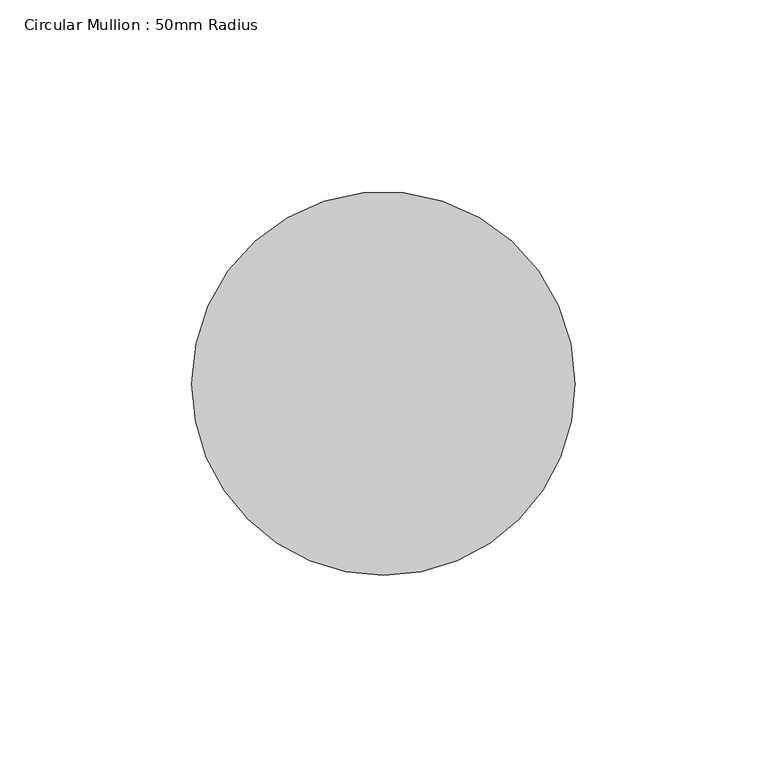
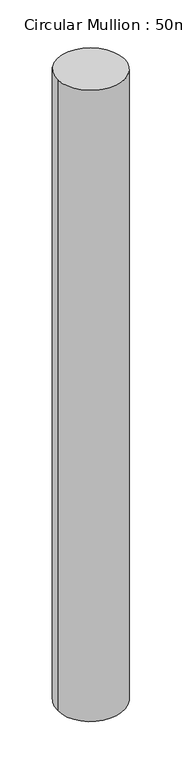
"""IFC4 building model written with IfcOpenShell, lengths in millimetres: member geometry, Circular Mullion : 50mm Radius."""

from ifc_helpers import new_model, si_unit, frame, origin, place, context, project, spatial, ellipse_curve, source, transform, mapped, element, save
from ifc_brep_helpers import plane_surface, cylinder_surface, advanced_brep


def circular_mullion_50mm_radius_109ee58a(model_context):
    return source(origin(), model_context, "Body", "AdvancedBrep", [
        advanced_brep(
        [(-100.0, 0.0, 1.7226691), (0.0, 0.0, 0.0), (0.0, 0.0, -1000.1450195), (-100.0, 0.0, -1001.858581)],
        [
            (0, 1, ellipse_curve(frame((-50.0, 0.0, 0.8613346), z_axis=(-0.017222365244023395, -0.014337637097104682, -0.9997488796182135), x_axis=(-0.7683427698041905, -0.6396461603007542, 0.022409321768563015)), 50.0125592, 50.0)),
            (1, 2),
            (2, 3, ellipse_curve(frame((-50.0, 0.0, -1001.0018003), z_axis=(-0.017131357412412482, -0.014261872982005232, 0.9997515269166901), x_axis=(0.7683448043477514, 0.6396478540603955, 0.022290904596866914)), 50.0124267, 50.0)),
            (3, 0),
            (1, 0, ellipse_curve(frame((-50.0, 0.0, 0.8613346), z_axis=(-0.017222365244023395, -0.014337637097104682, -0.9997488796182135), x_axis=(-0.7683427698041905, -0.6396461603007542, 0.022409321768563015)), 50.0125592, 50.0)),
            (3, 2, ellipse_curve(frame((-50.0, 0.0, -1001.0018003), z_axis=(-0.017131357412412482, -0.014261872982005232, 0.9997515269166901), x_axis=(0.7683448043477514, 0.6396478540603955, 0.022290904596866914)), 50.0124267, 50.0)),
        ],
        [
            cylinder_surface(frame((-50.0, 0.0, 0.0), z_axis=(0.0, 0.0, 1.0), x_axis=(1.0, 0.0, 0.0)), 50.0),
            plane_surface(frame((-195.0131214, 234.2497011, 0.0), z_axis=(0.0172223652440234, 0.014337637097104686, 0.9997488796182137), x_axis=(0.7683427698041908, 0.6396461603007537, -0.02240932176855912))),
            plane_surface(frame((-195.0131214, 234.2497011, -1000.1450195), z_axis=(0.017131357412412482, 0.014261872982005232, -0.9997515269166901), x_axis=(0.7683448043477515, 0.6396478540603953, 0.022290904596868))),
        ],
        [
            (0, [[1, 2, 3, 4]]),
            (0, [[5, -4, 6, -2]]),
            (1, [[-1, -5]]),
            (2, [[-6, -3]]),
        ],
    ),
    ])


if __name__ == "__main__":
    model = new_model("IFC4")
    model_context = context("Model", 3, world=origin())
    ifc_project = project(units=[si_unit("LENGTHUNIT", "METRE", prefix="MILLI")], contexts=[model_context])
    site = spatial("IfcSite", under=ifc_project)
    building = spatial("IfcBuilding", under=site)
    placement = place(None, origin())
    circular_mullion_50mm_radius_shape = circular_mullion_50mm_radius_109ee58a(model_context)
    element("IfcMember", 1, ObjectType="Circular Mullion : 50mm Radius", at=placement, inside=building, context=model_context, shape_type="MappedRepresentation", body=[
        mapped(circular_mullion_50mm_radius_shape, transform((0.0, 0.0, 0.0), x_axis=(1.0, 0.0, 0.0), y_axis=(0.0, 1.0, 0.0), z_axis=(0.0, 0.0, 1.0))),
    ])
    save(model, "model.ifc")

# Revit data of these elements
# Type "Circular Mullion : 50mm Radius"
#   built-in parameter 1007350 = 0.164042 (stored number, unit not read)
# Element 1 (IfcMember, "Circular Mullion : 50mm Radius")
#   Materials on its faces: "Aluminium"
# Materials
#   "Aluminium": class "Metal", colour RGB 247 247 247, transparency 0, Description = "Aluminium 6061", Cost = 0
